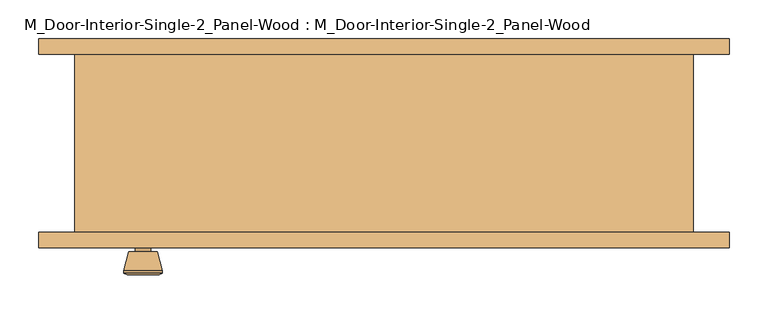
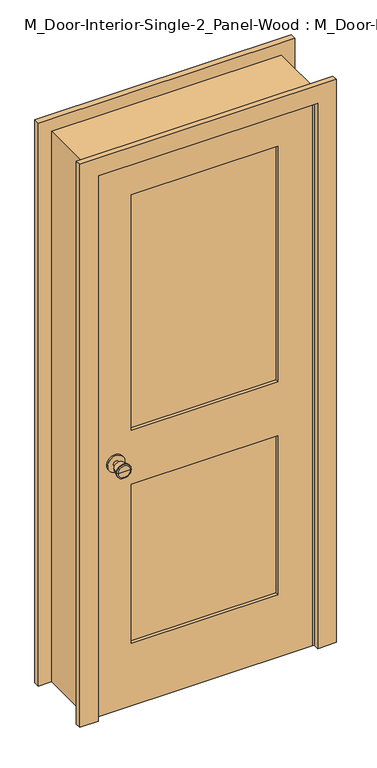
"""IFC4 building model written with IfcOpenShell, lengths in millimetres: door geometry, M_Door-Interior-Single-2_Panel-Wood : M_Door-Interior-Single-2_Panel-Wood."""

from ifc_helpers import new_model, si_unit, point, frame, frame_2d, origin, place, context, project, spatial, polyline, circle_curve, trimmed, segment, composite_curve, outline, extrude, faceted_brep, source, transform, mapped, element, save
from ifc_brep_helpers import plane_surface, cylinder_surface, revolved_surface, advanced_brep


def m_door_interior_single_2_panel_wood_m_door_interior_single_2_ce316a4d(model_context):
    return source(origin(), model_context, "Body", "SolidModel", [
        advanced_brep(
        [(-311.5, -70.825, 914.4), (-321.5, -70.825, 914.4), (-301.5, -70.825, 914.4), (-291.0241324, -21.825, 914.4), (-331.9758676, -21.825, 914.4), (-311.5, -21.825, 914.4), (-286.5, -23.6528681, 914.4), (-336.5, -23.6528681, 914.4), (-286.5, -27.1165463, 914.4), (-336.5, -27.1165463, 914.4), (-292.863764, -51.825, 914.4), (-330.136236, -51.825, 914.4), (-301.5, -51.825, 914.4), (-321.5, -51.825, 914.4)],
        [
            (0, 1),
            (1, 2, circle_curve(frame((-311.5, -70.825, 914.4), z_axis=(0.0, -1.0, 0.0), x_axis=(-1.0, 0.0, 0.0)), 10.0)),
            (2, 0),
            (2, 1, circle_curve(frame((-311.5, -70.825, 914.4), z_axis=(0.0, -1.0, 0.0), x_axis=(-1.0, 0.0, 0.0)), 10.0)),
            (3, 4, circle_curve(frame((-311.5, -21.825, 914.4), z_axis=(0.0, 1.0, 0.0), x_axis=(-1.0, 0.0, 0.0)), 20.4758676)),
            (4, 5),
            (5, 3),
            (4, 3, circle_curve(frame((-311.5, -21.825, 914.4), z_axis=(0.0, 1.0, 0.0), x_axis=(-1.0, 0.0, 0.0)), 20.4758676)),
            (6, 7, circle_curve(frame((-311.5, -23.6528681, 914.4), z_axis=(0.0, 1.0, 0.0), x_axis=(-1.0, 0.0, 0.0)), 25.0)),
            (7, 4),
            (3, 6),
            (7, 6, circle_curve(frame((-311.5, -23.6528681, 914.4), z_axis=(0.0, 1.0, 0.0), x_axis=(-1.0, 0.0, 0.0)), 25.0)),
            (8, 9, circle_curve(frame((-311.5, -27.1165463, 914.4), z_axis=(0.0, 1.0, 0.0), x_axis=(-1.0, 0.0, 0.0)), 25.0)),
            (9, 7),
            (6, 8),
            (9, 8, circle_curve(frame((-311.5, -27.1165463, 914.4), z_axis=(0.0, 1.0, 0.0), x_axis=(-1.0, 0.0, 0.0)), 25.0)),
            (10, 11, circle_curve(frame((-311.5, -51.825, 914.4), z_axis=(0.0, 1.0, 0.0), x_axis=(-1.0, 0.0, 0.0)), 18.636236)),
            (11, 9),
            (8, 10),
            (11, 10, circle_curve(frame((-311.5, -51.825, 914.4), z_axis=(0.0, 1.0, 0.0), x_axis=(-1.0, 0.0, 0.0)), 18.636236)),
            (12, 13, circle_curve(frame((-311.5, -51.825, 914.4), z_axis=(0.0, 1.0, 0.0), x_axis=(-1.0, 0.0, 0.0)), 10.0)),
            (13, 11),
            (10, 12),
            (13, 12, circle_curve(frame((-311.5, -51.825, 914.4), z_axis=(0.0, 1.0, 0.0), x_axis=(-1.0, 0.0, 0.0)), 10.0)),
            (1, 13),
            (12, 2),
        ],
        [
            plane_surface(frame((-311.5, -70.825, 914.4), z_axis=(0.0, -1.0, 0.0), x_axis=(-1.0, 0.0, 0.0))),
            plane_surface(frame((-311.5, -21.825, 914.4), z_axis=(0.0, 1.0, 0.0), x_axis=(-1.0, 0.0, 0.0))),
            revolved_surface(polyline([(-331.9758676, -21.825, 914.4), (-336.5, -23.6528681, 914.4)]), (-311.5, -70.825, 914.4), (0.0, -1.0, 0.0)),
            cylinder_surface(frame((-311.5, -70.825, 914.4), z_axis=(0.0, -1.0, 0.0), x_axis=(-1.0, 0.0, 0.0)), 25.0),
            revolved_surface(polyline([(-336.5, -27.1165463, 914.4), (-330.136236, -51.825, 914.4)]), (-311.5, -70.825, 914.4), (0.0, -1.0, 0.0)),
            plane_surface(frame((-311.5, -51.825, 914.4), z_axis=(0.0, -1.0, 0.0), x_axis=(-1.0, 0.0, 0.0))),
            cylinder_surface(frame((-311.5, -70.825, 914.4), z_axis=(0.0, -1.0, 0.0), x_axis=(-1.0, 0.0, 0.0)), 10.0),
        ],
        [
            (0, [[1, 2, 3]]),
            (0, [[-3, 4, -1]]),
            (1, [[5, 6, 7]]),
            (1, [[8, -7, -6]]),
            (2, [[9, 10, -5, 11]]),
            (2, [[12, -11, -8, -10]]),
            (3, [[13, 14, -9, 15]]),
            (3, [[16, -15, -12, -14]]),
            (4, [[17, 18, -13, 19]]),
            (4, [[20, -19, -16, -18]]),
            (5, [[21, 22, -17, 23]]),
            (5, [[24, -23, -20, -22]]),
            (6, [[-2, 25, -21, 26]]),
            (6, [[-4, -26, -24, -25]]),
        ],
    ),
        extrude(outline(composite_curve([segment(trimmed(circle_curve(frame_2d((914.4, -311.5)), 30.0), [point((914.4, -341.5))], [point((914.4, -281.5))], False, "CARTESIAN"), True, "CONTINUOUS"), segment(trimmed(circle_curve(frame_2d((914.4, -311.5)), 30.0), [point((914.4, -281.5))], [point((914.4, -341.5))], False, "CARTESIAN"), True, "CONTINUOUS")], self_intersect=False)), frame((0.0, -76.825, 0.0), z_axis=(0.0, 1.0, 0.0), x_axis=(0.0, 0.0, 1.0)), (0.0, 0.0, 1.0), 6.0),
        advanced_brep(
        [(-311.5, -117.825, 914.4), (-301.5, -117.825, 914.4), (-321.5, -117.825, 914.4), (-291.0241324, -166.825, 914.4), (-311.5, -166.825, 914.4), (-331.9758676, -166.825, 914.4), (-286.5, -164.9971319, 914.4), (-336.5, -164.9971319, 914.4), (-286.5, -161.5334537, 914.4), (-336.5, -161.5334537, 914.4), (-292.863764, -136.825, 914.4), (-330.136236, -136.825, 914.4), (-301.5, -136.825, 914.4), (-321.5, -136.825, 914.4)],
        [
            (0, 1),
            (1, 2, circle_curve(frame((-311.5, -117.825, 914.4), z_axis=(0.0, 1.0, 0.0), x_axis=(-1.0, 0.0, 0.0)), 10.0)),
            (2, 0),
            (2, 1, circle_curve(frame((-311.5, -117.825, 914.4), z_axis=(0.0, 1.0, 0.0), x_axis=(-1.0, 0.0, 0.0)), 10.0)),
            (3, 4),
            (4, 5),
            (5, 3, circle_curve(frame((-311.5, -166.825, 914.4), z_axis=(0.0, -1.0, 0.0), x_axis=(-1.0, 0.0, 0.0)), 20.4758676)),
            (3, 5, circle_curve(frame((-311.5, -166.825, 914.4), z_axis=(0.0, -1.0, 0.0), x_axis=(-1.0, 0.0, 0.0)), 20.4758676)),
            (6, 3),
            (5, 7),
            (7, 6, circle_curve(frame((-311.5, -164.9971319, 914.4), z_axis=(0.0, -1.0, 0.0), x_axis=(-1.0, 0.0, 0.0)), 25.0)),
            (6, 7, circle_curve(frame((-311.5, -164.9971319, 914.4), z_axis=(0.0, -1.0, 0.0), x_axis=(-1.0, 0.0, 0.0)), 25.0)),
            (8, 6),
            (7, 9),
            (9, 8, circle_curve(frame((-311.5, -161.5334537, 914.4), z_axis=(0.0, -1.0, 0.0), x_axis=(-1.0, 0.0, 0.0)), 25.0)),
            (8, 9, circle_curve(frame((-311.5, -161.5334537, 914.4), z_axis=(0.0, -1.0, 0.0), x_axis=(-1.0, 0.0, 0.0)), 25.0)),
            (10, 8),
            (9, 11),
            (11, 10, circle_curve(frame((-311.5, -136.825, 914.4), z_axis=(0.0, -1.0, 0.0), x_axis=(-1.0, 0.0, 0.0)), 18.636236)),
            (10, 11, circle_curve(frame((-311.5, -136.825, 914.4), z_axis=(0.0, -1.0, 0.0), x_axis=(-1.0, 0.0, 0.0)), 18.636236)),
            (12, 10),
            (11, 13),
            (13, 12, circle_curve(frame((-311.5, -136.825, 914.4), z_axis=(0.0, -1.0, 0.0), x_axis=(-1.0, 0.0, 0.0)), 10.0)),
            (12, 13, circle_curve(frame((-311.5, -136.825, 914.4), z_axis=(0.0, -1.0, 0.0), x_axis=(-1.0, 0.0, 0.0)), 10.0)),
            (1, 12),
            (13, 2),
        ],
        [
            plane_surface(frame((-311.5, -117.825, 914.4), z_axis=(0.0, 1.0, 0.0), x_axis=(-1.0, 0.0, 0.0))),
            plane_surface(frame((-311.5, -166.825, 914.4), z_axis=(0.0, -1.0, 0.0), x_axis=(-1.0, 0.0, 0.0))),
            revolved_surface(polyline([(-331.9758676, -166.825, 914.4), (-336.5, -164.9971319, 914.4)]), (-311.5, -117.825, 914.4), (0.0, 1.0, 0.0)),
            cylinder_surface(frame((-311.5, -117.825, 914.4), z_axis=(0.0, 1.0, 0.0), x_axis=(-1.0, 0.0, 0.0)), 25.0),
            revolved_surface(polyline([(-336.5, -161.5334537, 914.4), (-330.136236, -136.825, 914.4)]), (-311.5, -117.825, 914.4), (0.0, 1.0, 0.0)),
            plane_surface(frame((-311.5, -136.825, 914.4), z_axis=(0.0, 1.0, 0.0), x_axis=(-1.0, 0.0, 0.0))),
            cylinder_surface(frame((-311.5, -117.825, 914.4), z_axis=(0.0, 1.0, 0.0), x_axis=(-1.0, 0.0, 0.0)), 10.0),
        ],
        [
            (0, [[1, 2, 3]]),
            (0, [[-3, 4, -1]]),
            (1, [[5, 6, 7]]),
            (1, [[-6, -5, 8]]),
            (2, [[9, -7, 10, 11]]),
            (2, [[-10, -8, -9, 12]]),
            (3, [[13, -11, 14, 15]]),
            (3, [[-14, -12, -13, 16]]),
            (4, [[17, -15, 18, 19]]),
            (4, [[-18, -16, -17, 20]]),
            (5, [[21, -19, 22, 23]]),
            (5, [[-22, -20, -21, 24]]),
            (6, [[25, -23, 26, -2]]),
            (6, [[-26, -24, -25, -4]]),
        ],
    ),
        extrude(outline(composite_curve([segment(trimmed(circle_curve(frame_2d((914.4, -311.5)), 30.0), [point((914.4, -341.5))], [point((914.4, -281.5))], False, "CARTESIAN"), True, "CONTINUOUS"), segment(trimmed(circle_curve(frame_2d((914.4, -311.5)), 30.0), [point((914.4, -281.5))], [point((914.4, -341.5))], False, "CARTESIAN"), True, "CONTINUOUS")], self_intersect=False)), frame((0.0, -117.825, 0.0), z_axis=(0.0, 1.0, 0.0), x_axis=(0.0, 0.0, 1.0)), (0.0, 0.0, 1.0), 6.0),
        extrude(outline(polyline([(255.0, -88.4916667), (255.0, -100.1583333), (-255.0, -100.1583333), (-255.0, -88.4916667), (255.0, -88.4916667)])), frame((0.0, 0.0, 1014.4), z_axis=(0.0, 0.0, 1.0), x_axis=(1.0, 0.0, 0.0)), (0.0, 0.0, 1.0), 865.6),
        extrude(outline(polyline([(255.0, -88.4916667), (255.0, -100.1583333), (-255.0, -100.1583333), (-255.0, -88.4916667), (255.0, -88.4916667)])), frame((0.0, 0.0, 230.0), z_axis=(0.0, 0.0, 1.0), x_axis=(1.0, 0.0, 0.0)), (0.0, 0.0, 1.0), 584.4),
        extrude(outline(polyline([(2000.0, -375.0), (0.0, -375.0), (0.0, 375.0), (2000.0, 375.0), (2000.0, -375.0)]), holes=[polyline([(1880.0, -255.0), (1880.0, 255.0), (1014.4, 255.0), (1014.4, -255.0), (1880.0, -255.0)]), polyline([(814.4, -255.0), (814.4, 255.0), (230.0, 255.0), (230.0, -255.0), (814.4, -255.0)])]), frame((0.0, -111.825, 0.0), z_axis=(0.0, 1.0, 0.0), x_axis=(0.0, 0.0, 1.0)), (0.0, 0.0, 1.0), 35.0),
        faceted_brep([(400.0, -111.825, 0.0), (375.0, -111.825, 0.0), (375.0, -76.825, 0.0), (362.3, -76.825, 0.0), (362.3, -41.9, 0.0), (375.0, -41.9, 0.0), (375.0, 118.175, 0.0), (400.0, 118.175, 0.0), (400.0, 118.175, 2025.0), (400.0, -111.825, 2025.0), (375.0, 118.175, 2000.0), (-375.0, 118.175, 2000.0), (-375.0, 118.175, 0.0), (-400.0, 118.175, 0.0), (-400.0, 118.175, 2025.0), (375.0, -41.9, 2000.0), (362.3, -41.9, 1987.3), (-362.3, -41.9, 1987.3), (-362.3, -41.9, 0.0), (-375.0, -41.9, 0.0), (-375.0, -41.9, 2000.0), (362.3, -76.825, 1987.3), (375.0, -76.825, 2000.0), (-375.0, -76.825, 2000.0), (-375.0, -76.825, 0.0), (-362.3, -76.825, 0.0), (-362.3, -76.825, 1987.3), (375.0, -111.825, 2000.0), (-400.0, -111.825, 2025.0), (-400.0, -111.825, 0.0), (-375.0, -111.825, 0.0), (-375.0, -111.825, 2000.0)], [[[0, 1, 2, 3, 4, 5, 6, 7]], [[7, 8, 9, 0]], [[6, 10, 11, 12, 13, 14, 8, 7]], [[5, 15, 10, 6]], [[4, 16, 17, 18, 19, 20, 15, 5]], [[3, 21, 16, 4]], [[2, 22, 23, 24, 25, 26, 21, 3]], [[1, 27, 22, 2]], [[0, 9, 28, 29, 30, 31, 27, 1]], [[8, 14, 28, 9]], [[15, 20, 11, 10]], [[21, 26, 17, 16]], [[27, 31, 23, 22]], [[29, 13, 12, 19, 18, 25, 24, 30]], [[14, 13, 29, 28]], [[20, 19, 12, 11]], [[26, 25, 18, 17]], [[31, 30, 24, 23]]]),
        extrude(outline(polyline([(0.0, 446.35), (2071.35, 446.35), (2071.35, -446.35), (0.0, -446.35), (0.0, -381.35), (2006.35, -381.35), (2006.35, 381.35), (0.0, 381.35), (0.0, 446.35)])), frame((0.0, 118.175, 0.0), z_axis=(0.0, 1.0, 0.0), x_axis=(0.0, 0.0, 1.0)), (0.0, 0.0, 1.0), 20.0),
        extrude(outline(polyline([(0.0, 446.35), (2071.35, 446.35), (2071.35, -446.35), (0.0, -446.35), (0.0, -381.35), (2006.35, -381.35), (2006.35, 381.35), (0.0, 381.35), (0.0, 446.35)])), frame((0.0, -131.825, 0.0), z_axis=(0.0, 1.0, 0.0), x_axis=(0.0, 0.0, 1.0)), (0.0, 0.0, 1.0), 20.0),
    ])


if __name__ == "__main__":
    model = new_model("IFC4")
    model_context = context("Model", 3, world=origin())
    ifc_project = project(units=[si_unit("LENGTHUNIT", "METRE", prefix="MILLI")], contexts=[model_context])
    site = spatial("IfcSite", under=ifc_project)
    building = spatial("IfcBuilding", under=site)
    placement = place(None, origin())
    m_door_interior_single_2_panel_wood_m_door_interior_single_2_shape = m_door_interior_single_2_panel_wood_m_door_interior_single_2_ce316a4d(model_context)
    element("IfcDoor", 1, ObjectType="M_Door-Interior-Single-2_Panel-Wood : M_Door-Interior-Single-2_Panel-Wood", at=placement, inside=building, context=model_context, shape_type="MappedRepresentation", body=[
        mapped(m_door_interior_single_2_panel_wood_m_door_interior_single_2_shape, transform((0.0, 0.0, 0.0), x_axis=(1.0, 0.0, 0.0), y_axis=(0.0, 1.0, 0.0), z_axis=(0.0, 0.0, 1.0))),
    ])
    save(model, "model.ifc")

# Revit data of these elements
# Type "M_Door-Interior-Single-2_Panel-Wood : M_Door-Interior-Single-2_Panel-Wood"
#   Type Mark = "52"
#   Assembly Code = "C1020300"
#   Analytic Construction = "Wooden"
#   Top Rail = 0.12 m
#   Thickness = 0.035 m
#   Thermal Resistance (R) = 0.455703 (m²·K)/W
#   Swing Angle [instance default] = 90.00°
#   Stiles = 0.12 m
#   Rough Width = 0.8 m
#   Rough Height = 2.025 m
#   Lock Rail = 0.2 m
#   Height = 2 m
#   Width = 0.75 m
#   Heat Transfer Coefficient (U) = 2.19465 W/(m²·K)
#   Bottom Rail = 0.23 m
#   Trim Material = Cherry
#   Panel Material = Cherry
#   Frame Material = Cherry
#   Door Handle Material = Aluminum
#   Visual Light Transmittance = 0
#   Solar Heat Gain Coefficient = 0
#   Wall Closure = (empty or 0)
#   Function = (empty or 0)
# Element 1 (IfcDoor, "M_Door-Interior-Single-2_Panel-Wood : M_Door-Interior-Single-2_Panel-Wood")
#   Materials on its faces: "Cherry", "Aluminum"
# Materials
#   "Cherry": class "Wood", colour RGB 226 177 128, transparency 0, Description = "Prunus Serotina", Cost = 0
#   "Aluminum": class "Metal", colour RGB 247 247 247, transparency 0, Description = "Aluminum 6061", Cost = 0
